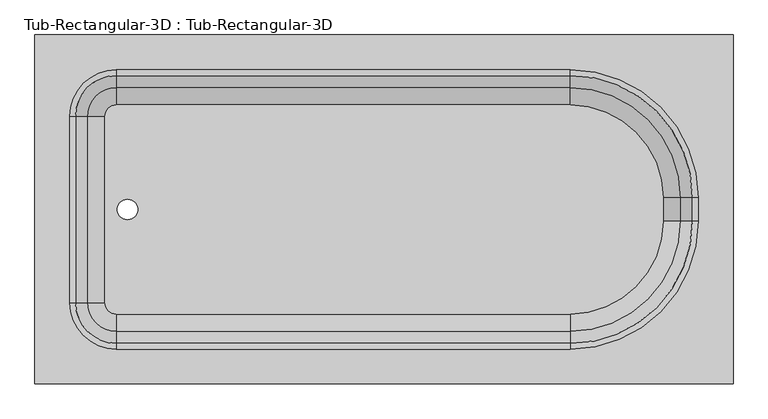
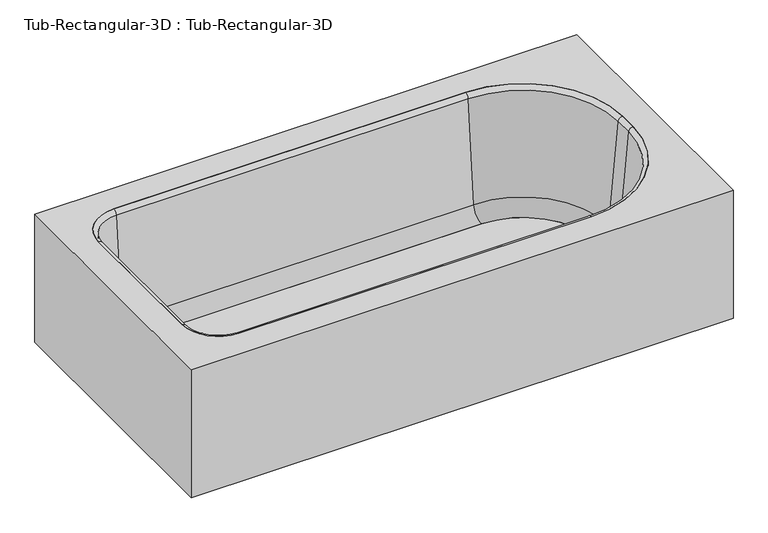
"""IFC4 building model written with IfcOpenShell, lengths in millimetres: flow terminal geometry, Tub-Rectangular-3D : Tub-Rectangular-3D."""

import ifcopenshell
import ifcopenshell.guid

model = None  # the IFC model being written
_history = None  # IfcOwnerHistory: only IFC2X3 demands one
_inside = {}  # id of a spatial element -> (the spatial element, [elements in it])
_under = {}  # id of a project, library or spatial element -> (it, [spatial elements below it])
_declared = {}  # id of a project -> (the project, [libraries it declares])
_typed = {}  # id of a type object -> (the type object, [elements of that type])
_made_of = {}  # id of a material, layer set ... -> (it, [elements and type objects made of it])


def new_model(schema):
    """Start an empty IFC model of exactly this schema.

    Asked for "IFC4X3", IfcOpenShell would pick the latest addendum, in which some entities
    have other attributes; the version numbers below select the first issue.
    IFC2X3 requires an IfcOwnerHistory on every rooted entity: one is made here for all.
    """
    global model, _history
    if schema == "IFC4X3":
        model = ifcopenshell.file(schema_version=(4, 3, 0, 0))
    else:
        model = ifcopenshell.file(schema=schema)
    _inside.clear()
    _under.clear()
    _declared.clear()
    _typed.clear()
    _made_of.clear()
    _history = None
    if model.schema == "IFC2X3":
        org = make("IfcOrganization", Name="unknown")
        user = make(
            "IfcPersonAndOrganization",
            ThePerson=make("IfcPerson", FamilyName="unknown"),
            TheOrganization=org,
        )
        app = make(
            "IfcApplication",
            ApplicationDeveloper=org,
            Version="unknown",
            ApplicationFullName="unknown",
            ApplicationIdentifier="unknown",
        )
        _history = make(
            "IfcOwnerHistory",
            OwningUser=user,
            OwningApplication=app,
            ChangeAction="ADDED",
            CreationDate=0,
        )
    return model


def make(cls, **values):
    """One entity of the class cls with the attributes given. An attribute that is None is left unset."""
    return model.create_entity(
        cls, **{name: value for name, value in values.items() if value is not None}
    )


def rooted(cls, **values):
    """An entity with a GlobalId (a new one), such as an element, a storey or a relation."""
    return make(cls, GlobalId=ifcopenshell.guid.new(), OwnerHistory=_history, **values)


def si_unit(unit_type, name, prefix=None):
    """IfcSIUnit, for example si_unit("LENGTHUNIT", "METRE", prefix="MILLI")."""
    return make("IfcSIUnit", UnitType=unit_type, Prefix=prefix, Name=name)


def assignment(units):
    """IfcUnitAssignment: the units of a project."""
    return None if units is None else make("IfcUnitAssignment", Units=units)


def point(xyz):
    """IfcCartesianPoint."""
    return None if xyz is None else make("IfcCartesianPoint", Coordinates=xyz)


def direction(xyz):
    """IfcDirection."""
    return None if xyz is None else make("IfcDirection", DirectionRatios=xyz)


def frame(location, z_axis=None, x_axis=None):
    """IfcAxis2Placement3D, a coordinate frame: its origin and axes. An axis left out is left unset."""
    return make(
        "IfcAxis2Placement3D",
        Location=point(location),
        Axis=direction(z_axis),
        RefDirection=direction(x_axis),
    )


def frame_2d(location, x_axis=None):
    """IfcAxis2Placement2D, a coordinate frame in the plane: its origin and x axis."""
    return make(
        "IfcAxis2Placement2D", Location=point(location), RefDirection=direction(x_axis)
    )


def origin():
    """The frame at (0, 0, 0) with its axes left unset."""
    return frame((0.0, 0.0, 0.0))


def place(relative_to, where):
    """IfcLocalPlacement: puts the frame where relative to a parent placement (None: the world)."""
    return make(
        "IfcLocalPlacement", PlacementRelTo=relative_to, RelativePlacement=where
    )


def context(
    kind, dimensions, precision=None, world=None, true_north=None, identifier=None
):
    """IfcGeometricRepresentationContext, for example the 3D "Model" context."""
    return make(
        "IfcGeometricRepresentationContext",
        ContextIdentifier=identifier,
        ContextType=kind,
        CoordinateSpaceDimension=dimensions,
        Precision=precision,
        WorldCoordinateSystem=world,
        TrueNorth=true_north,
    )


def project(units=None, contexts=None):
    """IfcProject with its units and contexts."""
    return rooted(
        "IfcProject",
        Name="project",
        RepresentationContexts=contexts,
        UnitsInContext=assignment(units),
    )


def spatial(cls, under=None, at=None, **own):
    """A site, building, storey or space (cls), placed at a placement, below another one or the project."""
    s = rooted(cls, ObjectPlacement=at, **own)
    if under is not None:
        _under.setdefault(under.id(), (under, []))[1].append(s)
    return s


def polyline(points):
    """IfcPolyline through the points."""
    return make("IfcPolyline", Points=[point(p) for p in points])


def circle_curve(where, radius):
    """IfcCircle in the frame where."""
    return make("IfcCircle", Position=where, Radius=radius)


def ellipse_curve(where, semi_axis1, semi_axis2):
    """IfcEllipse in the frame where."""
    return make(
        "IfcEllipse", Position=where, SemiAxis1=semi_axis1, SemiAxis2=semi_axis2
    )


def trimmed(basis, trim1, trim2, sense, master):
    """IfcTrimmedCurve: the piece of a basis curve between two trims."""
    return make(
        "IfcTrimmedCurve",
        BasisCurve=basis,
        Trim1=trim1,
        Trim2=trim2,
        SenseAgreement=sense,
        MasterRepresentation=master,
    )


def segment(curve, same_sense, transition):
    """IfcCompositeCurveSegment."""
    return make(
        "IfcCompositeCurveSegment",
        Transition=transition,
        SameSense=same_sense,
        ParentCurve=curve,
    )


def composite_curve(segments, self_intersect=None):
    """IfcCompositeCurve: segments joined end to end."""
    return make("IfcCompositeCurve", Segments=segments, SelfIntersect=self_intersect)


def outline(outer, holes=None, kind="AREA"):
    """IfcArbitraryClosedProfileDef: a profile drawn as a closed curve; with holes, ...WithVoids."""
    if holes is None:
        return make("IfcArbitraryClosedProfileDef", ProfileType=kind, OuterCurve=outer)
    return make(
        "IfcArbitraryProfileDefWithVoids",
        ProfileType=kind,
        OuterCurve=outer,
        InnerCurves=holes,
    )


def extrude(swept, where, along, depth):
    """IfcExtrudedAreaSolid: the profile swept, set in the frame where, extruded along a direction by depth."""
    return make(
        "IfcExtrudedAreaSolid",
        SweptArea=swept,
        Position=where,
        ExtrudedDirection=direction(along),
        Depth=depth,
    )


def shape(context_of_items, identifier, shape_type, items):
    """IfcShapeRepresentation: the items that make up one representation, for example the "Body"."""
    return make(
        "IfcShapeRepresentation",
        ContextOfItems=context_of_items,
        RepresentationIdentifier=identifier,
        RepresentationType=shape_type,
        Items=items,
    )


def source(mapping_origin, context_of_items, identifier, shape_type, items):
    """IfcRepresentationMap: a shape defined once, which mapped items show again and again."""
    return make(
        "IfcRepresentationMap",
        MappingOrigin=mapping_origin,
        MappedRepresentation=shape(context_of_items, identifier, shape_type, items),
    )


def transform(
    local_origin,
    x_axis=None,
    y_axis=None,
    z_axis=None,
    scale=None,
    scale2=None,
    scale3=None,
    uniform=True,
):
    """IfcCartesianTransformationOperator3D, or its non-uniform kind. x_axis, y_axis, z_axis: its Axis1, 2, 3."""
    if uniform:
        return make(
            "IfcCartesianTransformationOperator3D",
            Axis1=direction(x_axis),
            Axis2=direction(y_axis),
            LocalOrigin=point(local_origin),
            Scale=scale,
            Axis3=direction(z_axis),
        )
    return make(
        "IfcCartesianTransformationOperator3DnonUniform",
        Axis1=direction(x_axis),
        Axis2=direction(y_axis),
        LocalOrigin=point(local_origin),
        Scale=scale,
        Axis3=direction(z_axis),
        Scale2=scale2,
        Scale3=scale3,
    )


def mapped(mapping_source, mapping_target):
    """IfcMappedItem: shows the shape of a source again, moved by a transform."""
    return make(
        "IfcMappedItem", MappingSource=mapping_source, MappingTarget=mapping_target
    )


def made_of(thing, what):
    """Note that an element or type object is made of a material, layer set ...; save() writes the relation."""
    if what is not None:
        _made_of.setdefault(what.id(), (what, []))[1].append(thing)
    return thing


def element(
    cls,
    number,
    at=None,
    inside=None,
    cuts=None,
    type_object=None,
    material=None,
    context=None,
    identifier="Body",
    shape_type=None,
    held_by="IfcProductDefinitionShape",
    body=None,
    shapes=None,
    **own,
):
    """One element of the class cls, such as IfcWall. Its Tag is "e" and its number.

    at: its placement. inside: the storey or other place that contains it. cuts: it is an
    opening in that element (IfcRelVoidsElement). A single representation is given by context,
    identifier, shape_type and body (its items); several are given by shapes. held_by: the class
    of the entity that holds the representations. save() writes the other relations.
    """
    e = rooted(cls, Tag="e%d" % number, ObjectPlacement=at, **own)
    if body is not None:
        shapes = [shape(context, identifier, shape_type, body)]
    if shapes is not None:
        e.Representation = make(held_by, Representations=shapes)
    if inside is not None:
        _inside.setdefault(inside.id(), (inside, []))[1].append(e)
    if cuts is not None:
        rooted(
            "IfcRelVoidsElement", RelatingBuildingElement=cuts, RelatedOpeningElement=e
        )
    if type_object is not None:
        _typed.setdefault(type_object.id(), (type_object, []))[1].append(e)
    return made_of(e, material)


def aggregate(whole, parts):
    """IfcRelAggregates: a whole, such as a stair, and the parts it consists of."""
    return rooted("IfcRelAggregates", RelatingObject=whole, RelatedObjects=parts)


def save(model, path):
    """Write the relations noted so far, then the file.

    IfcRelAggregates (storeys below a building ...), IfcRelContainedInSpatialStructure (elements
    in a storey), IfcRelDefinesByType, IfcRelAssociatesMaterial and IfcRelDeclares: one each for
    every whole, place, type object, material and project.
    """
    for whole, parts in _under.values():
        aggregate(whole, parts)
    for where, things in _inside.values():
        rooted(
            "IfcRelContainedInSpatialStructure",
            RelatedElements=things,
            RelatingStructure=where,
        )
    for kind, things in _typed.values():
        rooted("IfcRelDefinesByType", RelatedObjects=things, RelatingType=kind)
    for what, things in _made_of.values():
        rooted("IfcRelAssociatesMaterial", RelatedObjects=things, RelatingMaterial=what)
    for by, libraries in _declared.values():
        rooted("IfcRelDeclares", RelatingContext=by, RelatedDefinitions=libraries)
    model.write(path)


def plane_surface(at):
    """IfcPlane: the flat surface through the origin of the frame at, square to its z axis."""
    return make("IfcPlane", Position=at)


def cylinder_surface(at, radius):
    """IfcCylindricalSurface: all points at the distance radius from the z axis of the frame at."""
    return make("IfcCylindricalSurface", Position=at, Radius=radius)


def revolved_surface(curve, axis_point, axis_direction):
    """IfcSurfaceOfRevolution: the curve turned about the line through axis_point along axis_direction."""
    return make(
        "IfcSurfaceOfRevolution",
        SweptCurve=make("IfcArbitraryOpenProfileDef", ProfileType="CURVE", Curve=curve),
        AxisPosition=make("IfcAxis1Placement", Location=point(axis_point), Axis=direction(axis_direction)),
    )


def advanced_brep(points, edges, surfaces, faces):
    """IfcAdvancedBrep: a solid bounded by faces that lie on surfaces and meet in shared edges.

    An edge is (start, end): straight between two places in points (the first is 0);
    or (start, end, curve); or (start, end, curve, False) where it runs against its curve.
    A face is (place in surfaces, loops), or (place, loops, False) where it looks against
    its surface's normal. A loop lists edges by number (the first is 1), with a minus sign
    where the edge is run from its end to its start. The first loop is the outer one.
    """
    corners = [point(p) for p in points]
    vertices = [make("IfcVertexPoint", VertexGeometry=c) for c in corners]
    made = []
    for start, end, *more in edges:
        made.append(
            make(
                "IfcEdgeCurve",
                EdgeStart=vertices[start],
                EdgeEnd=vertices[end],
                EdgeGeometry=more[0] if more else make("IfcPolyline", Points=[corners[start], corners[end]]),
                SameSense=more[1] if len(more) > 1 else True,
            )
        )
    hull = []
    for where, loops, *sense in faces:
        bounds = []
        for j, loop in enumerate(loops):
            ring = [make("IfcOrientedEdge", EdgeElement=made[abs(k) - 1], Orientation=k > 0) for k in loop]
            bounds.append(
                make(
                    "IfcFaceOuterBound" if j == 0 else "IfcFaceBound",
                    Bound=make("IfcEdgeLoop", EdgeList=ring),
                    Orientation=True,
                )
            )
        hull.append(make("IfcAdvancedFace", Bounds=bounds, FaceSurface=surfaces[where], SameSense=sense[0] if sense else True))
    return make("IfcAdvancedBrep", Outer=make("IfcClosedShell", CfsFaces=hull))


def tub_rectangular_3d_tub_rectangular_3d_50c8b8b2(model_context):
    return source(origin(), model_context, "Body", "SolidModel", [
        advanced_brep(
        [(413.3970313, 858.8375, 381.0), (-1110.6029687, 858.8375, 381.0), (-1110.6029687, 96.8375, 381.0), (413.3970313, 96.8375, 381.0), (-932.8029687, 782.6375, 381.0), (57.7970313, 782.6375, 381.0), (337.1970313, 503.2375, 381.0), (337.1970313, 452.4375, 381.0), (57.7970313, 173.0375, 381.0), (-932.8029687, 173.0375, 381.0), (-1034.4029687, 274.6375, 381.0), (-1034.4029687, 681.0375, 381.0), (394.3470313, 839.7875, 361.95), (394.3470313, 115.8875, 361.95), (-1091.5529687, 115.8875, 361.95), (-1091.5529687, 839.7875, 361.95), (-932.8029687, 782.6375, 361.95), (-1034.4029687, 681.0375, 361.95), (-1034.4029687, 274.6375, 361.95), (-932.8029687, 173.0375, 361.95), (57.7970313, 173.0375, 361.95), (337.1970313, 452.4375, 361.95), (337.1970313, 503.2375, 361.95), (57.7970313, 782.6375, 361.95), (413.3970313, 858.8375, 0.0), (-1110.6029687, 858.8375, 0.0), (-1110.6029687, 96.8375, 0.0), (413.3970313, 96.8375, 0.0), (394.3470313, 839.7875, 0.0), (-1091.5529687, 839.7875, 0.0), (-1091.5529687, 115.8875, 0.0), (394.3470313, 115.8875, 0.0)],
        [
            (0, 1),
            (1, 2),
            (2, 3),
            (3, 0),
            (4, 5),
            (5, 6, circle_curve(frame((57.7970313, 503.2375, 381.0), z_axis=(0.0, 0.0, -1.0), x_axis=(0.0, 1.0, 0.0)), 279.4)),
            (6, 7),
            (7, 8, circle_curve(frame((57.7970313, 452.4375, 381.0), z_axis=(0.0, 0.0, -1.0), x_axis=(0.0, 1.0, 0.0)), 279.4)),
            (8, 9),
            (9, 10, circle_curve(frame((-932.8029687, 274.6375, 381.0), z_axis=(0.0, 0.0, -1.0), x_axis=(0.0, 1.0, 0.0)), 101.6)),
            (10, 11),
            (11, 4, circle_curve(frame((-932.8029687, 681.0375, 381.0), z_axis=(0.0, 0.0, -1.0), x_axis=(0.0, 1.0, 0.0)), 101.6)),
            (12, 13),
            (13, 14),
            (14, 15),
            (15, 12),
            (16, 17, circle_curve(frame((-932.8029687, 681.0375, 361.95), z_axis=(0.0, 0.0, 1.0), x_axis=(0.0, 1.0, 0.0)), 101.6)),
            (17, 18),
            (18, 19, circle_curve(frame((-932.8029687, 274.6375, 361.95), z_axis=(0.0, 0.0, 1.0), x_axis=(0.0, 1.0, 0.0)), 101.6)),
            (19, 20),
            (20, 21, circle_curve(frame((57.7970313, 452.4375, 361.95), z_axis=(0.0, 0.0, 1.0), x_axis=(0.0, 1.0, 0.0)), 279.4)),
            (21, 22),
            (22, 23, circle_curve(frame((57.7970313, 503.2375, 361.95), z_axis=(0.0, 0.0, 1.0), x_axis=(0.0, 1.0, 0.0)), 279.4)),
            (23, 16),
            (0, 24),
            (24, 25),
            (25, 1),
            (25, 26),
            (26, 2),
            (26, 27),
            (27, 3),
            (27, 24),
            (4, 16),
            (23, 5),
            (22, 6),
            (21, 7),
            (20, 8),
            (19, 9),
            (18, 10),
            (17, 11),
            (28, 29),
            (29, 30),
            (30, 31),
            (31, 28),
            (31, 13),
            (12, 28),
            (30, 14),
            (29, 15),
        ],
        [
            plane_surface(frame((-1110.6029687, 858.8375, 381.0), z_axis=(0.0, 0.0, 1.0), x_axis=(-1.0, 0.0, 0.0))),
            plane_surface(frame((-1110.6029687, 858.8375, 361.95), z_axis=(0.0, 0.0, -1.0), x_axis=(1.0, 0.0, 0.0))),
            plane_surface(frame((413.3970313, 858.8375, 381.0), z_axis=(0.0, 1.0, 0.0), x_axis=(0.0, 0.0, -1.0))),
            plane_surface(frame((-1110.6029687, 858.8375, 381.0), z_axis=(-1.0, 0.0, 0.0), x_axis=(0.0, 0.0, -1.0))),
            plane_surface(frame((-1110.6029687, 96.8375, 381.0), z_axis=(0.0, -1.0, 0.0), x_axis=(0.0, 0.0, -1.0))),
            plane_surface(frame((413.3970313, 96.8375, 381.0), z_axis=(1.0, 0.0, 0.0), x_axis=(0.0, 0.0, -1.0))),
            plane_surface(frame((-932.8029687, 782.6375, 381.0), z_axis=(0.0, -1.0, 0.0), x_axis=(0.0, 0.0, -1.0))),
            revolved_surface(polyline([(57.7970313, 782.6375, 361.95), (57.7970313, 782.6375, 381.0)]), (57.7970313, 503.2375, 381.0), (0.0, 0.0, -1.0)),
            plane_surface(frame((337.1970313, 503.2375, 381.0), z_axis=(-1.0, 0.0, 0.0), x_axis=(0.0, 0.0, -1.0))),
            revolved_surface(polyline([(57.7970313, 731.8375, 361.95), (57.7970313, 731.8375, 381.0)]), (57.7970313, 452.4375, 381.0), (0.0, 0.0, -1.0)),
            plane_surface(frame((57.7970313, 173.0375, 381.0), z_axis=(0.0, 1.0, 0.0), x_axis=(0.0, 0.0, -1.0))),
            revolved_surface(polyline([(-932.8029687, 376.23749999999995, 361.95), (-932.8029687, 376.23749999999995, 381.0)]), (-932.8029687, 274.6375, 381.0), (0.0, 0.0, -1.0)),
            plane_surface(frame((-1034.4029687, 274.6375, 381.0), z_axis=(1.0, 0.0, 0.0), x_axis=(0.0, 0.0, -1.0))),
            revolved_surface(polyline([(-932.8029687, 782.6375, 361.95), (-932.8029687, 782.6375, 381.0)]), (-932.8029687, 681.0375, 381.0), (0.0, 0.0, -1.0)),
            plane_surface(frame((-1110.6029687, 858.8375, 0.0), z_axis=(0.0, 0.0, -1.0), x_axis=(1.0, 0.0, 0.0))),
            plane_surface(frame((394.3470313, 839.7875, 361.95), z_axis=(-1.0, 0.0, 0.0), x_axis=(0.0, 0.0, -1.0))),
            plane_surface(frame((394.3470313, 115.8875, 361.95), z_axis=(0.0, 1.0, 0.0), x_axis=(0.0, 0.0, -1.0))),
            plane_surface(frame((-1091.5529687, 115.8875, 361.95), z_axis=(1.0, 0.0, 0.0), x_axis=(0.0, 0.0, -1.0))),
            plane_surface(frame((-1091.5529687, 839.7875, 361.95), z_axis=(0.0, -1.0, 0.0), x_axis=(0.0, 0.0, -1.0))),
        ],
        [
            (0, [[1, 2, 3, 4], [5, 6, 7, 8, 9, 10, 11, 12]]),
            (1, [[13, 14, 15, 16], [17, 18, 19, 20, 21, 22, 23, 24]]),
            (2, [[-1, 25, 26, 27]]),
            (3, [[-2, -27, 28, 29]]),
            (4, [[-3, -29, 30, 31]]),
            (5, [[-25, -4, -31, 32]]),
            (6, [[-5, 33, -24, 34]]),
            (7, [[-6, -34, -23, 35]]),
            (8, [[-7, -35, -22, 36]]),
            (9, [[-8, -36, -21, 37]]),
            (10, [[-9, -37, -20, 38]]),
            (11, [[-10, -38, -19, 39]]),
            (12, [[-11, -39, -18, 40]]),
            (13, [[-12, -40, -17, -33]]),
            (14, [[-32, -30, -28, -26], [41, 42, 43, 44]]),
            (15, [[-44, 45, -13, 46]]),
            (16, [[-43, 47, -14, -45]]),
            (17, [[-42, 48, -15, -47]]),
            (18, [[-41, -46, -16, -48]]),
        ],
    ),
        extrude(outline(composite_curve([segment(trimmed(circle_curve(frame_2d((57.7970313, 503.2375)), 202.7964741), [point((57.7970313, 706.0339741))], [point((260.5935054, 503.2375))], False, "CARTESIAN"), True, "CONTINUOUS"), segment(polyline([(260.5935054, 503.2375), (260.5935054, 452.4375)]), True, "CONTINUOUS"), segment(trimmed(circle_curve(frame_2d((57.7970313, 452.4375)), 202.7964741), [point((260.5935054, 452.4375))], [point((57.7970313, 249.6410259))], False, "CARTESIAN"), True, "CONTINUOUS"), segment(polyline([(57.7970313, 249.6410259), (-932.8029687, 249.6410259)]), True, "CONTINUOUS"), segment(trimmed(circle_curve(frame_2d((-932.8029687, 274.6375)), 24.9964741), [point((-932.8029687, 249.6410259))], [point((-957.7994428, 274.6375))], False, "CARTESIAN"), True, "CONTINUOUS"), segment(polyline([(-957.7994428, 274.6375), (-957.7994428, 681.0375)]), True, "CONTINUOUS"), segment(trimmed(circle_curve(frame_2d((-932.8029687, 681.0375)), 24.9964741), [point((-957.7994428, 681.0375))], [point((-932.8029687, 706.0339741))], False, "CARTESIAN"), True, "CONTINUOUS"), segment(polyline([(-932.8029687, 706.0339741), (57.7970313, 706.0339741)]), True, "CONTINUOUS")], self_intersect=False), holes=[composite_curve([segment(trimmed(circle_curve(frame_2d((-908.510206, 477.8375)), 22.225), [point((-908.510206, 500.0625))], [point((-908.510206, 455.6125))], True, "CARTESIAN"), True, "CONTINUOUS"), segment(trimmed(circle_curve(frame_2d((-908.510206, 477.8375)), 22.225), [point((-908.510206, 455.6125))], [point((-908.510206, 500.0625))], True, "CARTESIAN"), True, "CONTINUOUS")], self_intersect=False)]), frame((0.0, 0.0, 16.863573), z_axis=(0.0, 0.0, 1.0), x_axis=(1.0, 0.0, 0.0)), (0.0, 0.0, 1.0), 19.05),
        advanced_brep(
        [(-995.7544608, 681.0375, 70.6929392), (-932.8029687, 743.9889921, 70.6929392), (-932.8029687, 770.1595035, 369.8232535), (-1021.9249722, 681.0375, 369.8232535), (-957.7994428, 681.0375, 35.913573), (-932.8029687, 706.0339741, 35.913573), (-957.7994428, 681.0375, 16.863573), (-932.8029687, 706.0339741, 16.863573), (-1034.4029687, 681.0375, 16.863573), (-932.8029687, 782.6375, 16.863573), (-1034.4029687, 681.0375, 381.0), (-932.8029687, 782.6375, 381.0), (-1021.9249722, 274.6375, 369.8232535), (-995.7544608, 274.6375, 70.6929392), (-957.7994428, 274.6375, 35.913573), (-957.7994428, 274.6375, 16.863573), (-1034.4029687, 274.6375, 16.863573), (-1034.4029687, 274.6375, 381.0), (-932.8029687, 211.6860079, 70.6929392), (-932.8029687, 185.5154965, 369.8232535), (-932.8029687, 249.6410259, 35.913573), (-932.8029687, 249.6410259, 16.863573), (-932.8029687, 173.0375, 16.863573), (-932.8029687, 173.0375, 381.0), (57.7970313, 185.5154965, 369.8232535), (57.7970313, 211.6860079, 70.6929392), (57.7970313, 249.6410259, 35.913573), (57.7970313, 249.6410259, 16.863573), (57.7970313, 173.0375, 16.863573), (57.7970313, 173.0375, 381.0), (298.5485234, 452.4375, 70.6929392), (324.7190348, 452.4375, 369.8232535), (260.5935054, 452.4375, 35.913573), (260.5935054, 452.4375, 16.863573), (337.1970313, 452.4375, 16.863573), (337.1970313, 452.4375, 381.0), (324.7190348, 503.2375, 369.8232535), (298.5485234, 503.2375, 70.6929392), (260.5935054, 503.2375, 35.913573), (260.5935054, 503.2375, 16.863573), (337.1970313, 503.2375, 16.863573), (337.1970313, 503.2375, 381.0), (57.7970313, 743.9889921, 70.6929392), (57.7970313, 770.1595035, 369.8232535), (57.7970313, 706.0339741, 35.913573), (57.7970313, 706.0339741, 16.863573), (57.7970313, 782.6375, 16.863573), (57.7970313, 782.6375, 381.0)],
        [
            (0, 1, circle_curve(frame((-932.8029687, 681.0375, 70.6929392), z_axis=(0.0, 0.0, -1.0), x_axis=(0.0, 1.0, 0.0)), 62.9514921)),
            (1, 2),
            (2, 3, circle_curve(frame((-932.8029687, 681.0375, 369.8232535), z_axis=(0.0, 0.0, 1.0), x_axis=(0.0, 1.0, 0.0)), 89.1220035)),
            (3, 0),
            (4, 5, circle_curve(frame((-932.8029687, 681.0375, 35.913573), z_axis=(0.0, 0.0, -1.0), x_axis=(0.0, 1.0, 0.0)), 24.9964741)),
            (5, 1, circle_curve(frame((-932.8029687, 706.0339741, 74.013573), z_axis=(1.0, 0.0, 0.0), x_axis=(0.0, -1.0, 0.0)), 38.1)),
            (0, 4, circle_curve(frame((-957.7994428, 681.0375, 74.013573), z_axis=(0.0, -1.0, 0.0), x_axis=(1.0, 0.0, 0.0)), 38.1)),
            (6, 7, circle_curve(frame((-932.8029687, 681.0375, 16.863573), z_axis=(0.0, 0.0, -1.0), x_axis=(0.0, 1.0, 0.0)), 24.9964741)),
            (7, 5),
            (4, 6),
            (8, 9, circle_curve(frame((-932.8029687, 681.0375, 16.863573), z_axis=(0.0, 0.0, -1.0), x_axis=(0.0, 1.0, 0.0)), 101.6)),
            (9, 7),
            (6, 8),
            (10, 11, circle_curve(frame((-932.8029687, 681.0375, 381.0), z_axis=(0.0, 0.0, -1.0), x_axis=(0.0, 1.0, 0.0)), 101.6)),
            (11, 9),
            (8, 10),
            (2, 11, circle_curve(frame((-932.8029687, 782.6375, 368.4462547), z_axis=(-1.0, 0.0, 0.0), x_axis=(0.0, -1.0, 0.0)), 12.5537453)),
            (10, 3, circle_curve(frame((-1034.4029687, 681.0375, 368.4462547), z_axis=(0.0, 1.0, 0.0), x_axis=(1.0, 0.0, 0.0)), 12.5537453)),
            (3, 12),
            (12, 13),
            (13, 0),
            (13, 14, circle_curve(frame((-957.7994428, 274.6375, 74.013573), z_axis=(0.0, -1.0, 0.0), x_axis=(1.0, 0.0, 0.0)), 38.1)),
            (14, 4),
            (14, 15),
            (15, 6),
            (15, 16),
            (16, 8),
            (16, 17),
            (17, 10),
            (17, 12, circle_curve(frame((-1034.4029687, 274.6375, 368.4462547), z_axis=(0.0, 1.0, 0.0), x_axis=(1.0, 0.0, 0.0)), 12.5537453)),
            (18, 13, circle_curve(frame((-932.8029687, 274.6375, 70.6929392), z_axis=(0.0, 0.0, -1.0), x_axis=(-1.0, 0.0, 0.0)), 62.9514921)),
            (12, 19, circle_curve(frame((-932.8029687, 274.6375, 369.8232535), z_axis=(0.0, 0.0, 1.0), x_axis=(-1.0, 0.0, 0.0)), 89.1220035)),
            (19, 18),
            (20, 14, circle_curve(frame((-932.8029687, 274.6375, 35.913573), z_axis=(0.0, 0.0, -1.0), x_axis=(-1.0, 0.0, 0.0)), 24.9964741)),
            (18, 20, circle_curve(frame((-932.8029687, 249.6410259, 74.013573), z_axis=(1.0, 0.0, 0.0), x_axis=(0.0, 1.0, 0.0)), 38.1)),
            (21, 15, circle_curve(frame((-932.8029687, 274.6375, 16.863573), z_axis=(0.0, 0.0, -1.0), x_axis=(-1.0, 0.0, 0.0)), 24.9964741)),
            (20, 21),
            (22, 16, circle_curve(frame((-932.8029687, 274.6375, 16.863573), z_axis=(0.0, 0.0, -1.0), x_axis=(-1.0, 0.0, 0.0)), 101.6)),
            (21, 22),
            (23, 17, circle_curve(frame((-932.8029687, 274.6375, 381.0), z_axis=(0.0, 0.0, -1.0), x_axis=(-1.0, 0.0, 0.0)), 101.6)),
            (22, 23),
            (23, 19, circle_curve(frame((-932.8029687, 173.0375, 368.4462547), z_axis=(-1.0, 0.0, 0.0), x_axis=(0.0, 1.0, 0.0)), 12.5537453)),
            (19, 24),
            (24, 25),
            (25, 18),
            (25, 26, circle_curve(frame((57.7970313, 249.6410259, 74.013573), z_axis=(1.0, 0.0, 0.0), x_axis=(0.0, 1.0, 0.0)), 38.1)),
            (26, 20),
            (26, 27),
            (27, 21),
            (27, 28),
            (28, 22),
            (28, 29),
            (29, 23),
            (29, 24, circle_curve(frame((57.7970313, 173.0375, 368.4462547), z_axis=(-1.0, 0.0, 0.0), x_axis=(0.0, 1.0, 0.0)), 12.5537453)),
            (30, 25, circle_curve(frame((57.7970313, 452.4375, 70.6929392), z_axis=(0.0, 0.0, -1.0), x_axis=(0.0, -1.0, 0.0)), 240.7514921)),
            (24, 31, circle_curve(frame((57.7970313, 452.4375, 369.8232535), z_axis=(0.0, 0.0, 1.0), x_axis=(0.0, -1.0, 0.0)), 266.9220035)),
            (31, 30),
            (32, 26, circle_curve(frame((57.7970313, 452.4375, 35.913573), z_axis=(0.0, 0.0, -1.0), x_axis=(0.0, -1.0, 0.0)), 202.7964741)),
            (30, 32, circle_curve(frame((260.5935054, 452.4375, 74.013573), z_axis=(0.0, 1.0, 0.0), x_axis=(-1.0, 0.0, 0.0)), 38.1)),
            (33, 27, circle_curve(frame((57.7970313, 452.4375, 16.863573), z_axis=(0.0, 0.0, -1.0), x_axis=(0.0, -1.0, 0.0)), 202.7964741)),
            (32, 33),
            (34, 28, circle_curve(frame((57.7970313, 452.4375, 16.863573), z_axis=(0.0, 0.0, -1.0), x_axis=(0.0, -1.0, 0.0)), 279.4)),
            (33, 34),
            (35, 29, circle_curve(frame((57.7970313, 452.4375, 381.0), z_axis=(0.0, 0.0, -1.0), x_axis=(0.0, -1.0, 0.0)), 279.4)),
            (34, 35),
            (35, 31, circle_curve(frame((337.1970313, 452.4375, 368.4462547), z_axis=(0.0, -1.0, 0.0), x_axis=(-1.0, 0.0, 0.0)), 12.5537453)),
            (31, 36),
            (36, 37),
            (37, 30),
            (37, 38, circle_curve(frame((260.5935054, 503.2375, 74.013573), z_axis=(0.0, 1.0, 0.0), x_axis=(-1.0, 0.0, 0.0)), 38.1)),
            (38, 32),
            (38, 39),
            (39, 33),
            (39, 40),
            (40, 34),
            (40, 41),
            (41, 35),
            (41, 36, circle_curve(frame((337.1970313, 503.2375, 368.4462547), z_axis=(0.0, -1.0, 0.0), x_axis=(-1.0, 0.0, 0.0)), 12.5537453)),
            (42, 37, circle_curve(frame((57.7970313, 503.2375, 70.6929392), z_axis=(0.0, 0.0, -1.0), x_axis=(1.0, 0.0, 0.0)), 240.7514921)),
            (36, 43, circle_curve(frame((57.7970313, 503.2375, 369.8232535), z_axis=(0.0, 0.0, 1.0), x_axis=(1.0, 0.0, 0.0)), 266.9220035)),
            (43, 42),
            (44, 38, circle_curve(frame((57.7970313, 503.2375, 35.913573), z_axis=(0.0, 0.0, -1.0), x_axis=(1.0, 0.0, 0.0)), 202.7964741)),
            (42, 44, circle_curve(frame((57.7970313, 706.0339741, 74.013573), z_axis=(-1.0, 0.0, 0.0), x_axis=(0.0, -1.0, 0.0)), 38.1)),
            (45, 39, circle_curve(frame((57.7970313, 503.2375, 16.863573), z_axis=(0.0, 0.0, -1.0), x_axis=(1.0, 0.0, 0.0)), 202.7964741)),
            (44, 45),
            (46, 40, circle_curve(frame((57.7970313, 503.2375, 16.863573), z_axis=(0.0, 0.0, -1.0), x_axis=(1.0, 0.0, 0.0)), 279.4)),
            (45, 46),
            (47, 41, circle_curve(frame((57.7970313, 503.2375, 381.0), z_axis=(0.0, 0.0, -1.0), x_axis=(1.0, 0.0, 0.0)), 279.4)),
            (46, 47),
            (47, 43, circle_curve(frame((57.7970313, 782.6375, 368.4462547), z_axis=(1.0, 0.0, 0.0), x_axis=(0.0, -1.0, 0.0)), 12.5537453)),
            (43, 2),
            (1, 42),
            (5, 44),
            (7, 45),
            (9, 46),
            (11, 47),
        ],
        [
            revolved_surface(polyline([(-932.8029687, 770.1595035, 369.8232535), (-932.8029687, 743.9889921, 70.6929392)]), (-932.8029687, 681.0375, 381.0), (0.0, 0.0, 1.0)),
            revolved_surface(trimmed(ellipse_curve(frame((-932.8029687, 706.0339741, 74.013573), z_axis=(-1.0, 0.0, 0.0), x_axis=(0.0, -1.0, 0.0)), 38.1, 38.1), [point((-932.8029687, 743.9889921, 70.6929392))], [point((-932.8029687, 706.0339741, 35.913573))], True, "CARTESIAN"), (-932.8029687, 681.0375, 381.0), (0.0, 0.0, 1.0)),
            revolved_surface(polyline([(-932.8029687, 706.0339741, 35.913572999999985), (-932.8029687, 706.0339741, 16.863572999999974)]), (-932.8029687, 681.0375, 381.0), (0.0, 0.0, 1.0)),
            plane_surface(frame((-932.8029687, 681.0375, 16.863573), z_axis=(0.0, 0.0, -1.0), x_axis=(0.0, 1.0, 0.0))),
            cylinder_surface(frame((-932.8029687, 681.0375, 381.0), z_axis=(0.0, 0.0, 1.0), x_axis=(0.0, 1.0, 0.0)), 101.6),
            revolved_surface(trimmed(ellipse_curve(frame((-932.8029687, 782.6375, 368.4462547), z_axis=(1.0, 0.0, 0.0), x_axis=(0.0, -1.0, 0.0)), 12.5537453, 12.5537453), [point((-932.8029687, 782.6375, 381.0))], [point((-932.8029687, 770.1595035, 369.8232535))], True, "CARTESIAN"), (-932.8029687, 681.0375, 381.0), (0.0, 0.0, 1.0)),
            plane_surface(frame((-1021.9249722, 681.0375, 369.8232535), z_axis=(0.9961946980917458, 0.0, 0.08715574274765589), x_axis=(0.0, -1.0, 0.0))),
            revolved_surface(polyline([(-919.6994427999999, 274.6375, 74.013573), (-919.6994427999999, 681.0375, 74.013573)]), (-957.7994428, 681.0375, 74.013573), (0.0, -1.0, 0.0)),
            plane_surface(frame((-957.7994428, 681.0375, 35.913573), z_axis=(1.0, 0.0, 0.0), x_axis=(0.0, -1.0, 0.0))),
            plane_surface(frame((-957.7994428, 681.0375, 16.863573), z_axis=(0.0, 0.0, -1.0), x_axis=(0.0, -1.0, 0.0))),
            plane_surface(frame((-1034.4029687, 681.0375, 16.863573), z_axis=(-1.0, 0.0, 0.0), x_axis=(0.0, -1.0, 0.0))),
            cylinder_surface(frame((-1034.4029687, 681.0375, 368.4462547), z_axis=(0.0, 1.0, 0.0), x_axis=(1.0, 0.0, 0.0)), 12.5537453),
            revolved_surface(polyline([(-1021.9249722, 274.6375, 369.8232535), (-995.7544608, 274.6375, 70.6929392)]), (-932.8029687, 274.6375, 381.0), (0.0, 0.0, 1.0)),
            revolved_surface(trimmed(ellipse_curve(frame((-957.7994428, 274.6375, 74.013573), z_axis=(0.0, -1.0, 0.0), x_axis=(1.0, 0.0, 0.0)), 38.1, 38.1), [point((-995.7544608, 274.6375, 70.6929392))], [point((-957.7994428, 274.6375, 35.913573))], True, "CARTESIAN"), (-932.8029687, 274.6375, 381.0), (0.0, 0.0, 1.0)),
            revolved_surface(polyline([(-957.7994428, 274.6375, 35.913572999999985), (-957.7994428, 274.6375, 16.863572999999974)]), (-932.8029687, 274.6375, 381.0), (0.0, 0.0, 1.0)),
            plane_surface(frame((-932.8029687, 274.6375, 16.863573), z_axis=(0.0, 0.0, -1.0), x_axis=(-1.0, 0.0, 0.0))),
            cylinder_surface(frame((-932.8029687, 274.6375, 381.0), z_axis=(0.0, 0.0, 1.0), x_axis=(-1.0, 0.0, 0.0)), 101.6),
            revolved_surface(trimmed(ellipse_curve(frame((-1034.4029687, 274.6375, 368.4462547), z_axis=(0.0, 1.0, 0.0), x_axis=(1.0, 0.0, 0.0)), 12.5537453, 12.5537453), [point((-1034.4029687, 274.6375, 381.0))], [point((-1021.9249722, 274.6375, 369.8232535))], True, "CARTESIAN"), (-932.8029687, 274.6375, 381.0), (0.0, 0.0, 1.0)),
            plane_surface(frame((-932.8029687, 185.5154965, 369.8232535), z_axis=(0.0, 0.9961946980917461, 0.08715574274765266), x_axis=(1.0, 0.0, 0.0))),
            revolved_surface(polyline([(57.79703129999996, 287.7410259, 74.013573), (-932.8029687, 287.7410259, 74.013573)]), (-932.8029687, 249.6410259, 74.013573), (1.0, 0.0, 0.0)),
            plane_surface(frame((-932.8029687, 249.6410259, 35.913573), z_axis=(0.0, 1.0, 0.0), x_axis=(1.0, 0.0, 0.0))),
            plane_surface(frame((-932.8029687, 249.6410259, 16.863573), z_axis=(0.0, 0.0, -1.0), x_axis=(1.0, 0.0, 0.0))),
            plane_surface(frame((-932.8029687, 173.0375, 16.863573), z_axis=(0.0, -1.0, 0.0), x_axis=(1.0, 0.0, 0.0))),
            cylinder_surface(frame((-932.8029687, 173.0375, 368.4462547), z_axis=(-1.0, 0.0, 0.0), x_axis=(0.0, 1.0, 0.0)), 12.5537453),
            revolved_surface(polyline([(57.7970313, 185.5154965, 369.8232535), (57.7970313, 211.6860079, 70.6929392)]), (57.7970313, 452.4375, 381.0), (0.0, 0.0, 1.0)),
            revolved_surface(trimmed(ellipse_curve(frame((57.7970313, 249.6410259, 74.013573), z_axis=(1.0, 0.0, 0.0), x_axis=(0.0, 1.0, 0.0)), 38.1, 38.1), [point((57.7970313, 211.6860079, 70.6929392))], [point((57.7970313, 249.6410259, 35.913573))], True, "CARTESIAN"), (57.7970313, 452.4375, 381.0), (0.0, 0.0, 1.0)),
            revolved_surface(polyline([(57.7970313, 249.6410259, 35.913572999999985), (57.7970313, 249.6410259, 16.863572999999974)]), (57.7970313, 452.4375, 381.0), (0.0, 0.0, 1.0)),
            plane_surface(frame((57.7970313, 452.4375, 16.863573), z_axis=(0.0, 0.0, -1.0), x_axis=(0.0, -1.0, 0.0))),
            cylinder_surface(frame((57.7970313, 452.4375, 381.0), z_axis=(0.0, 0.0, 1.0), x_axis=(0.0, -1.0, 0.0)), 279.4),
            revolved_surface(trimmed(ellipse_curve(frame((57.7970313, 173.0375, 368.4462547), z_axis=(-1.0, 0.0, 0.0), x_axis=(0.0, 1.0, 0.0)), 12.5537453, 12.5537453), [point((57.7970313, 173.0375, 381.0))], [point((57.7970313, 185.5154965, 369.8232535))], True, "CARTESIAN"), (57.7970313, 452.4375, 381.0), (0.0, 0.0, 1.0)),
            plane_surface(frame((324.7190348, 452.4375, 369.8232535), z_axis=(-0.9961946980917464, 0.0, 0.08715574274764942), x_axis=(0.0, 1.0, 0.0))),
            revolved_surface(polyline([(222.49350540000003, 503.2375, 74.013573), (222.49350540000003, 452.4375, 74.013573)]), (260.5935054, 452.4375, 74.013573), (0.0, 1.0, 0.0)),
            plane_surface(frame((260.5935054, 452.4375, 35.913573), z_axis=(-1.0, 0.0, 0.0), x_axis=(0.0, 1.0, 0.0))),
            plane_surface(frame((260.5935054, 452.4375, 16.863573), z_axis=(0.0, 0.0, -1.0), x_axis=(0.0, 1.0, 0.0))),
            plane_surface(frame((337.1970313, 452.4375, 16.863573), z_axis=(1.0, 0.0, 0.0), x_axis=(0.0, 1.0, 0.0))),
            cylinder_surface(frame((337.1970313, 452.4375, 368.4462547), z_axis=(0.0, -1.0, 0.0), x_axis=(-1.0, 0.0, 0.0)), 12.5537453),
            revolved_surface(polyline([(324.7190348, 503.2375, 369.8232535), (298.5485234, 503.2375, 70.6929392)]), (57.7970313, 503.2375, 381.0), (0.0, 0.0, 1.0)),
            revolved_surface(trimmed(ellipse_curve(frame((260.5935054, 503.2375, 74.013573), z_axis=(0.0, 1.0, 0.0), x_axis=(-1.0, 0.0, 0.0)), 38.1, 38.1), [point((298.5485234, 503.2375, 70.6929392))], [point((260.5935054, 503.2375, 35.913573))], True, "CARTESIAN"), (57.7970313, 503.2375, 381.0), (0.0, 0.0, 1.0)),
            revolved_surface(polyline([(260.5935054, 503.2375, 35.913572999999985), (260.5935054, 503.2375, 16.863572999999974)]), (57.7970313, 503.2375, 381.0), (0.0, 0.0, 1.0)),
            plane_surface(frame((57.7970313, 503.2375, 16.863573), z_axis=(0.0, 0.0, -1.0), x_axis=(1.0, 0.0, 0.0))),
            cylinder_surface(frame((57.7970313, 503.2375, 381.0), z_axis=(0.0, 0.0, 1.0), x_axis=(1.0, 0.0, 0.0)), 279.4),
            revolved_surface(trimmed(ellipse_curve(frame((337.1970313, 503.2375, 368.4462547), z_axis=(0.0, -1.0, 0.0), x_axis=(-1.0, 0.0, 0.0)), 12.5537453, 12.5537453), [point((337.1970313, 503.2375, 381.0))], [point((324.7190348, 503.2375, 369.8232535))], True, "CARTESIAN"), (57.7970313, 503.2375, 381.0), (0.0, 0.0, 1.0)),
            plane_surface(frame((57.7970313, 770.1595035, 369.8232535), z_axis=(0.0, -0.9961946980917461, 0.08715574274765266), x_axis=(-1.0, 0.0, 0.0))),
            revolved_surface(polyline([(-932.8029687, 667.9339741, 74.013573), (57.7970313, 667.9339741, 74.013573)]), (57.7970313, 706.0339741, 74.013573), (-1.0, 0.0, 0.0)),
            plane_surface(frame((57.7970313, 706.0339741, 35.913573), z_axis=(0.0, -1.0, 0.0), x_axis=(-1.0, 0.0, 0.0))),
            plane_surface(frame((57.7970313, 706.0339741, 16.863573), z_axis=(0.0, 0.0, -1.0), x_axis=(-1.0, 0.0, 0.0))),
            plane_surface(frame((57.7970313, 782.6375, 16.863573), z_axis=(0.0, 1.0, 0.0), x_axis=(-1.0, 0.0, 0.0))),
            cylinder_surface(frame((57.7970313, 782.6375, 368.4462547), z_axis=(1.0, 0.0, 0.0), x_axis=(0.0, -1.0, 0.0)), 12.5537453),
        ],
        [
            (0, [[1, 2, 3, 4]]),
            (1, [[5, 6, -1, 7]]),
            (2, [[8, 9, -5, 10]]),
            (3, [[11, 12, -8, 13]]),
            (4, [[14, 15, -11, 16]]),
            (5, [[-3, 17, -14, 18]]),
            (6, [[-4, 19, 20, 21]]),
            (7, [[-7, -21, 22, 23]]),
            (8, [[-10, -23, 24, 25]]),
            (9, [[-13, -25, 26, 27]]),
            (10, [[-16, -27, 28, 29]]),
            (11, [[-18, -29, 30, -19]]),
            (12, [[31, -20, 32, 33]]),
            (13, [[34, -22, -31, 35]]),
            (14, [[36, -24, -34, 37]]),
            (15, [[38, -26, -36, 39]]),
            (16, [[40, -28, -38, 41]]),
            (17, [[-32, -30, -40, 42]]),
            (18, [[-33, 43, 44, 45]]),
            (19, [[-35, -45, 46, 47]]),
            (20, [[-37, -47, 48, 49]]),
            (21, [[-39, -49, 50, 51]]),
            (22, [[-41, -51, 52, 53]]),
            (23, [[-42, -53, 54, -43]]),
            (24, [[55, -44, 56, 57]]),
            (25, [[58, -46, -55, 59]]),
            (26, [[60, -48, -58, 61]]),
            (27, [[62, -50, -60, 63]]),
            (28, [[64, -52, -62, 65]]),
            (29, [[-56, -54, -64, 66]]),
            (30, [[-57, 67, 68, 69]]),
            (31, [[-59, -69, 70, 71]]),
            (32, [[-61, -71, 72, 73]]),
            (33, [[-63, -73, 74, 75]]),
            (34, [[-65, -75, 76, 77]]),
            (35, [[-66, -77, 78, -67]]),
            (36, [[79, -68, 80, 81]]),
            (37, [[82, -70, -79, 83]]),
            (38, [[84, -72, -82, 85]]),
            (39, [[86, -74, -84, 87]]),
            (40, [[88, -76, -86, 89]]),
            (41, [[-80, -78, -88, 90]]),
            (42, [[-81, 91, -2, 92]]),
            (43, [[-83, -92, -6, 93]]),
            (44, [[-85, -93, -9, 94]]),
            (45, [[-87, -94, -12, 95]]),
            (46, [[-89, -95, -15, 96]]),
            (47, [[-90, -96, -17, -91]]),
        ],
    ),
    ])


if __name__ == "__main__":
    model = new_model("IFC4")
    model_context = context("Model", 3, world=origin())
    ifc_project = project(units=[si_unit("LENGTHUNIT", "METRE", prefix="MILLI")], contexts=[model_context])
    site = spatial("IfcSite", under=ifc_project)
    building = spatial("IfcBuilding", under=site)
    placement = place(None, origin())
    tub_rectangular_3d_tub_rectangular_3d_shape = tub_rectangular_3d_tub_rectangular_3d_50c8b8b2(model_context)
    element("IfcFlowTerminal", 1, ObjectType="Tub-Rectangular-3D : Tub-Rectangular-3D", at=placement, inside=building, context=model_context, shape_type="MappedRepresentation", body=[
        mapped(tub_rectangular_3d_tub_rectangular_3d_shape, transform((0.0, 0.0, 0.0), x_axis=(1.0, 0.0, 0.0), y_axis=(0.0, 1.0, 0.0), z_axis=(0.0, 0.0, 1.0))),
    ])
    save(model, "model.ifc")

# Revit data of these elements
# Type "Tub-Rectangular-3D : Tub-Rectangular-3D"
#   Assembly Code = "D2010500"
#   Depth = 2' - 6"
#   Height = 1' - 3"
#   Width = 5' - 0"
#   Tub Material = Porcelain, Ivory
#   Default Elevation = 0
# Element 1 (IfcFlowTerminal, "Tub-Rectangular-3D : Tub-Rectangular-3D")
#   Materials on its faces: "Porcelain, Ivory"
# Materials
#   "Porcelain, Ivory": class "Ceramic", colour RGB 224 216 188, transparency 0, Description = "Porcelain, ivory", Cost = 0
